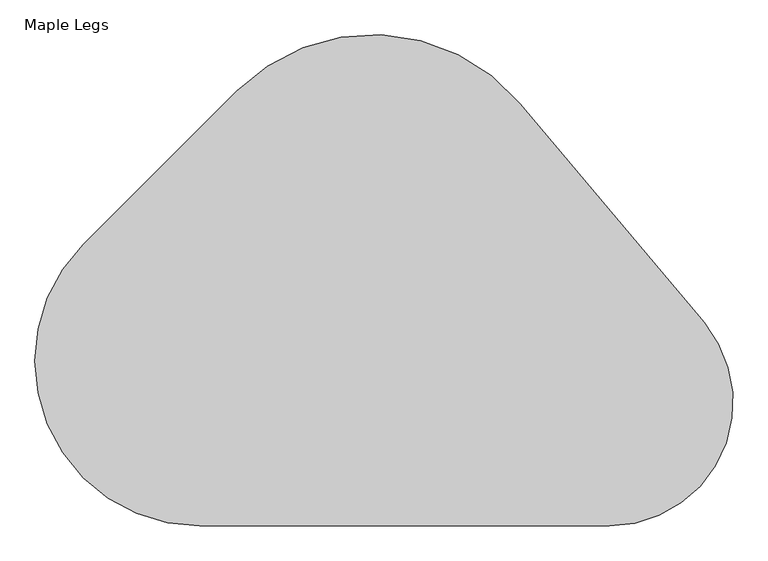
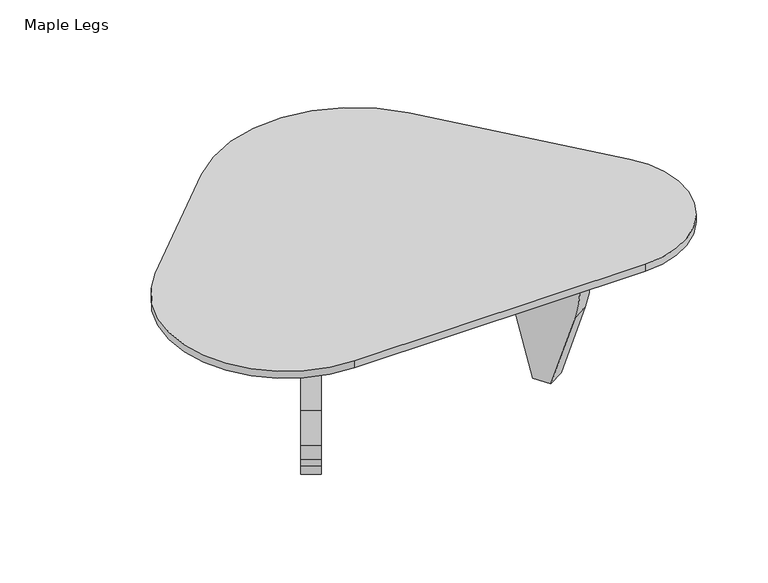
"""IFC4 building model written with IfcOpenShell, lengths in millimetres: furniture geometry, Noguchi Table : Maple Legs."""

from ifc_helpers import new_model, si_unit, point, frame, frame_2d, origin, place, context, project, spatial, polyline, circle_curve, trimmed, segment, composite_curve, outline, extrude, source, transform, mapped, element, save


def maple_legs_1e4ba76a(model_context):
    return source(origin(), model_context, "Body", "SweptSolid", [
        extrude(outline(composite_curve([segment(polyline([(-616.1982593, 166.2408792), (-332.9683375, 449.470801)]), True, "CONTINUOUS"), segment(trimmed(circle_curve(frame_2d((-81.5211661, 198.0236296)), 355.6), [point((-332.9683375, 449.470801))], [point((190.8842378, 426.5989036))], False, "CARTESIAN"), True, "CONTINUOUS"), segment(polyline([(190.8842378, 426.5989036), (530.8395157, 21.4559798)]), True, "CONTINUOUS"), segment(trimmed(circle_curve(frame_2d((355.721756, -125.4852677)), 228.6), [point((530.8395157, 21.4559798))], [point((355.721756, -354.0852677))], False, "CARTESIAN"), True, "CONTINUOUS"), segment(polyline([(355.721756, -354.0852677), (-400.6721124, -354.0852677)]), True, "CONTINUOUS"), segment(trimmed(circle_curve(frame_2d((-400.6721124, -49.2852677)), 304.8), [point((-400.6721124, -354.0852677))], [point((-616.1982593, 166.2408792))], False, "CARTESIAN"), True, "CONTINUOUS")], self_intersect=False)), frame((0.0, 0.0, 387.35), z_axis=(0.0, 0.0, 1.0), x_axis=(1.0, 0.0, 0.0)), (0.0, 0.0, 1.0), 19.05),
        extrude(outline(composite_curve([segment(trimmed(circle_curve(frame_2d((0.0, -292.1)), 292.1), [point((-85.401775, -12.7633808))], [point((0.0, 0.0))], False, "CARTESIAN"), True, "CONTINUOUS"), segment(polyline([(0.0, 0.0), (38.515049, 0.0)]), True, "CONTINUOUS"), segment(trimmed(circle_curve(frame_2d((38.515049, -44.45)), 44.45), [point((38.515049, 0.0))], [point((60.740049, -5.9551709))], False, "CARTESIAN"), True, "CONTINUOUS"), segment(polyline([(60.740049, -5.9551709), (99.9621328, -28.6000515), (99.9621328, -759.2112915), (61.6824096, -776.3453752)]), True, "CONTINUOUS"), segment(trimmed(circle_curve(frame_2d((46.368836, -742.1329034)), 37.4833132), [point((61.6824096, -776.3453752))], [point((46.368836, -779.6162166))], False, "CARTESIAN"), True, "CONTINUOUS"), segment(polyline([(46.368836, -779.6162166), (25.3127237, -779.6162166)]), True, "CONTINUOUS"), segment(trimmed(circle_curve(frame_2d((25.3127237, -684.3662165)), 95.25), [point((25.3127237, -779.6162166))], [point((-29.3204318, -762.3904488))], False, "CARTESIAN"), True, "CONTINUOUS"), segment(polyline([(-29.3204318, -762.3904488), (-93.5973313, -717.3832793), (-93.5973313, -679.2832792), (-37.9691113, -612.9881482)]), True, "CONTINUOUS"), segment(trimmed(circle_curve(frame_2d((-149.8499022, -519.1090178)), 146.05), [point((-37.9691113, -612.9881482))], [point((-3.7999022, -519.1090178))], True, "CARTESIAN"), True, "CONTINUOUS"), segment(polyline([(-3.7999022, -519.1090178), (-3.7999022, -289.2152929)]), True, "CONTINUOUS"), segment(trimmed(circle_curve(frame_2d((-124.4499022, -289.2152929)), 120.65), [point((-3.7999022, -289.2152929))], [point((-93.2233844, -172.6763419))], True, "CARTESIAN"), True, "CONTINUOUS"), segment(polyline([(-93.2233844, -172.6763419), (-287.3878672, -120.6501256), (-287.3878672, -74.5167265), (-85.401775, -12.7633808)]), True, "CONTINUOUS")], self_intersect=False)), frame((267.2461488, -214.3653004, 287.3878672), z_axis=(0.8480480961564271, 0.5299192642332033, 0.0), x_axis=(0.0, 0.0, 1.0)), (0.0, 0.0, 1.0), 48.5804754),
        extrude(outline(composite_curve([segment(trimmed(circle_curve(frame_2d((0.0, -292.1)), 292.1), [point((85.401775, -571.4366192))], [point((0.0, -584.2))], False, "CARTESIAN"), True, "CONTINUOUS"), segment(polyline([(0.0, -584.2), (-38.515049, -584.2)]), True, "CONTINUOUS"), segment(trimmed(circle_curve(frame_2d((-38.515049, -539.75)), 44.45), [point((-38.515049, -584.2))], [point((-60.740049, -578.2448292))], False, "CARTESIAN"), True, "CONTINUOUS"), segment(polyline([(-60.740049, -578.2448292), (-99.9621328, -555.5999486), (-99.9621328, 175.0112914), (-61.6824096, 192.1453752)]), True, "CONTINUOUS"), segment(trimmed(circle_curve(frame_2d((-46.368836, 157.9329033)), 37.4833132), [point((-61.6824096, 192.1453752))], [point((-46.368836, 195.4162165))], False, "CARTESIAN"), True, "CONTINUOUS"), segment(polyline([(-46.368836, 195.4162165), (-25.3127237, 195.4162165)]), True, "CONTINUOUS"), segment(trimmed(circle_curve(frame_2d((-25.3127237, 100.1662165)), 95.25), [point((-25.3127237, 195.4162165))], [point((29.3204318, 178.1904487))], False, "CARTESIAN"), True, "CONTINUOUS"), segment(polyline([(29.3204318, 178.1904487), (93.5973313, 133.1832792), (93.5973313, 95.0832791), (37.9691113, 28.7881481)]), True, "CONTINUOUS"), segment(trimmed(circle_curve(frame_2d((149.8499022, -65.0909823)), 146.05), [point((37.9691113, 28.7881481))], [point((3.7999022, -65.0909823))], True, "CARTESIAN"), True, "CONTINUOUS"), segment(polyline([(3.7999022, -65.0909823), (3.7999022, -291.9391371)]), True, "CONTINUOUS"), segment(trimmed(circle_curve(frame_2d((124.4499022, -291.9391371)), 120.65), [point((3.7999022, -291.9391371))], [point((93.2233844, -408.4780881))], True, "CARTESIAN"), True, "CONTINUOUS"), segment(polyline([(93.2233844, -408.4780881), (287.3878672, -460.5043044), (287.3878672, -509.6832736), (85.401775, -571.4366192)]), True, "CONTINUOUS")], self_intersect=False)), frame((-118.8687691, 281.4236, 99.9621328), z_axis=(-0.8660254037844366, 0.5000000000000038, 0.0), x_axis=(0.0, 0.0, 1.0)), (0.0, 0.0, 1.0), 46.6647559),
    ])


if __name__ == "__main__":
    model = new_model("IFC4")
    model_context = context("Model", 3, world=origin())
    ifc_project = project(units=[si_unit("LENGTHUNIT", "METRE", prefix="MILLI")], contexts=[model_context])
    site = spatial("IfcSite", under=ifc_project)
    building = spatial("IfcBuilding", under=site)
    placement = place(None, origin())
    maple_legs_shape = maple_legs_1e4ba76a(model_context)
    element("IfcFurniture", 1, ObjectType="Noguchi Table : Maple Legs", at=placement, inside=building, context=model_context, shape_type="MappedRepresentation", body=[
        mapped(maple_legs_shape, transform((0.0, 0.0, 0.0), x_axis=(1.0, 0.0, 0.0), y_axis=(0.0, 1.0, 0.0), z_axis=(0.0, 0.0, 1.0))),
    ])
    save(model, "model.ifc")

# Revit data of these elements
# Type "Noguchi Table : Maple Legs"
#   Leg Material = Wood - Cherry
# Element 1 (IfcFurniture, "Noguchi Table : Maple Legs")
#   Materials on its faces: "Wood - Cherry", "Glass"
# Materials
#   "Wood - Cherry": class "Wood", colour RGB 192 120 57, transparency 0, Comments = "Rendering appearance not upgraded Rendering appearance not upgraded ", Description = "Cherry"
#   "Glass": class "Glass", colour RGB 218 227 224, transparency 0.7, Comments = "Rendering appearance not upgraded Rendering appearance not upgraded ", Description = "Glass"
